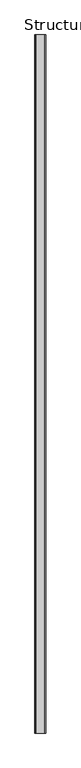
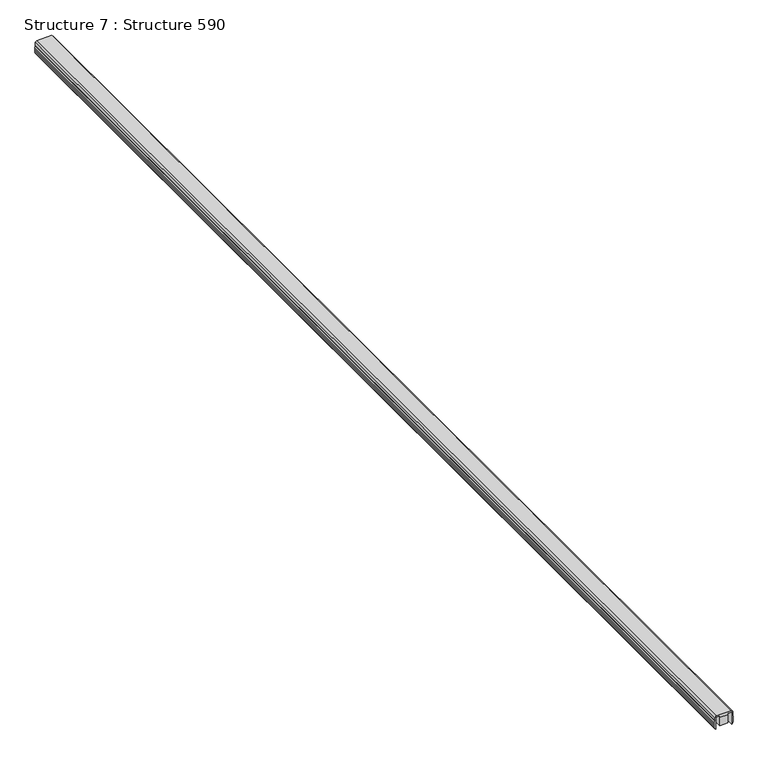
"""IFC4 building model written with IfcOpenShell, lengths in millimetres: proxy geometry, Structure 7 : Structure 590."""

from ifc_helpers import new_model, si_unit, frame, origin, place, context, project, spatial, polyline, outline, extrude, source, transform, mapped, element, save


def structure_7_structure_590_ca023d0f(model_context):
    return source(origin(), model_context, "Body", "SweptSolid", [
        extrude(outline(polyline([(39518.6052323, 7571.6095342), (39516.0973628, 7569.1016647), (39511.2956147, 7569.1016647), (39509.4309187, 7569.5762356), (39506.7561917, 7568.7736177), (39506.7561917, 7569.5762356), (39504.0814647, 7568.7736177), (39504.0814647, 7569.5762356), (39501.4067377, 7568.7736177), (39501.4067377, 7569.5762356), (39498.7320107, 7568.7736177), (39498.7320107, 7569.5762356), (39496.0572836, 7569.5762356), (39494.2728422, 7571.360677), (39515.9104029, 7571.360677), (39515.9104029, 7577.710677), (39513.3076045, 7577.710677), (39513.3076045, 7591.5121935), (39515.9104029, 7591.5121935), (39515.9104029, 7597.8621935), (39494.2728422, 7597.8621935), (39496.0572836, 7599.646635), (39498.7320107, 7599.646635), (39498.7320107, 7600.4492528), (39501.4067377, 7599.646635), (39501.4067377, 7600.4492528), (39504.0814647, 7599.646635), (39504.0814647, 7600.4492528), (39506.7561917, 7599.646635), (39506.7561917, 7600.4492528), (39509.4309187, 7599.646635), (39511.2956147, 7600.1212059), (39516.0973628, 7600.1212059), (39518.6052323, 7597.6133363), (39518.6052323, 7571.6095342)])), frame((0.0, -3747.9491938, 0.0), z_axis=(0.0, 1.0, 0.0), x_axis=(0.0, 0.0, 1.0)), (0.0, 0.0, 1.0), 2000.0),
        extrude(outline(polyline([(7591.5121935, -3747.9491938), (7577.710677, -3747.9491938), (7577.710677, -1747.9491938), (7591.5121935, -1747.9491938), (7591.5121935, -3747.9491938)])), frame((0.0, 0.0, 39498.7320107), z_axis=(0.0, 0.0, 1.0), x_axis=(1.0, 0.0, 0.0)), (0.0, 0.0, 1.0), 14.5755939),
    ])


if __name__ == "__main__":
    model = new_model("IFC4")
    model_context = context("Model", 3, world=origin())
    ifc_project = project(units=[si_unit("LENGTHUNIT", "METRE", prefix="MILLI")], contexts=[model_context])
    site = spatial("IfcSite", under=ifc_project)
    building = spatial("IfcBuilding", under=site)
    placement = place(None, origin())
    structure_7_structure_590_shape = structure_7_structure_590_ca023d0f(model_context)
    element("IfcBuildingElementProxy", 1, Name="Structure 7 : Structure 590", ObjectType="Structure 7 : Structure 590", at=placement, inside=building, context=model_context, shape_type="MappedRepresentation", body=[
        mapped(structure_7_structure_590_shape, transform((0.0, 0.0, 0.0), x_axis=(1.0, 0.0, 0.0), y_axis=(0.0, 1.0, 0.0), z_axis=(0.0, 0.0, 1.0))),
    ])
    save(model, "model.ifc")

# Revit data of these elements
# Type "Structure 7 : Structure 590"
#   NameOverride = "Structure"
# Element 1 (IfcBuildingElementProxy, "Structure 7 : Structure 590")
#   Materials on its faces: "RUBBER", "IfcSurfaceStyle #584"
# Materials
#   "RUBBER": class "Unassigned", colour RGB 70 70 70, transparency 0, Cost = 0
#   "IfcSurfaceStyle #584": class "Unassigned", colour RGB 169 181 186, transparency 0
